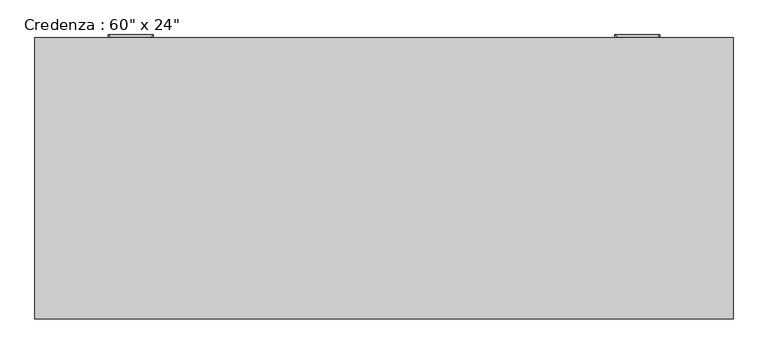
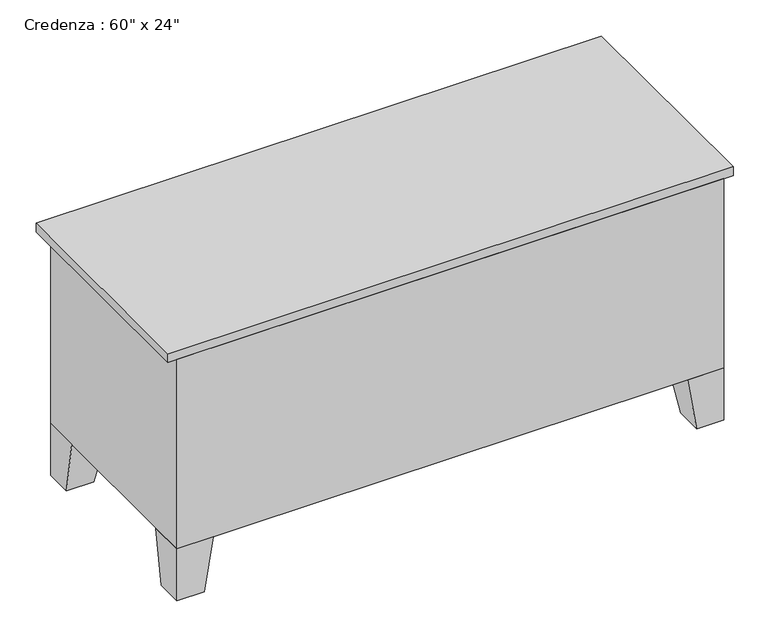
"""IFC4 building model written with IfcOpenShell, lengths in millimetres: furniture geometry."""

from ifc_helpers import new_model, si_unit, frame, origin, place, context, project, spatial, polyline, outline, extrude, faceted_brep, source, transform, mapped, element, save


def furniture_2f1724fb(model_context):
    return source(origin(), model_context, "Body", "SolidModel", [
        extrude(outline(polyline([(455.5023176, 267.2714583), (455.5023176, 254.5714583), (46.8442623, 254.5714583), (46.8442623, 267.2714583), (455.5023176, 267.2714583)])), frame((0.0, 0.0, 171.45), z_axis=(0.0, 0.0, 1.0), x_axis=(1.0, 0.0, 0.0)), (0.0, 0.0, 1.0), 520.7),
        extrude(outline(polyline([(73.6254475, 279.9714583), (73.6254475, 267.2714583), (-302.4057377, 267.2714583), (-302.4057377, 279.9714583), (73.6254475, 279.9714583)])), frame((0.0, 0.0, 171.45), z_axis=(0.0, 0.0, 1.0), x_axis=(1.0, 0.0, 0.0)), (0.0, 0.0, 1.0), 520.7),
        faceted_brep([(719.9442623, -309.3803279, 152.4), (821.5442623, -309.3803279, 152.4), (821.5442623, -207.7803279, 152.4), (719.9442623, -207.7803279, 152.4), (745.3442623, -309.3803279, 0.0), (745.3442623, -233.1803279, 0.0), (821.5442623, -233.1803279, 0.0), (821.5442623, -309.3803279, 0.0)], [[[0, 1, 2, 3]], [[4, 5, 6, 7]], [[4, 0, 3, 5]], [[5, 3, 2, 6]], [[6, 2, 1, 7]], [[7, 1, 0, 4]]]),
        extrude(outline(polyline([(802.4942623, 306.5696721), (802.4942623, 300.2196721), (440.5442623, 300.2196721), (440.5442623, 306.5696721), (802.4942623, 306.5696721)])), frame((0.0, 0.0, 584.2), z_axis=(0.0, 0.0, 1.0), x_axis=(1.0, 0.0, 0.0)), (0.0, 0.0, 1.0), 107.95),
        extrude(outline(polyline([(802.4942623, 306.5696721), (802.4942623, 300.2196721), (440.5442623, 300.2196721), (440.5442623, 306.5696721), (802.4942623, 306.5696721)])), frame((0.0, 0.0, 171.45), z_axis=(0.0, 0.0, 1.0), x_axis=(1.0, 0.0, 0.0)), (0.0, 0.0, 1.0), 393.7),
        extrude(outline(polyline([(-321.4557377, 306.5696721), (-321.4557377, 300.2196721), (-683.4057377, 300.2196721), (-683.4057377, 306.5696721), (-321.4557377, 306.5696721)])), frame((0.0, 0.0, 584.2), z_axis=(0.0, 0.0, 1.0), x_axis=(1.0, 0.0, 0.0)), (0.0, 0.0, 1.0), 107.95),
        extrude(outline(polyline([(-321.4557377, 306.5696721), (-321.4557377, 300.2196721), (-683.4057377, 300.2196721), (-683.4057377, 306.5696721), (-321.4557377, 306.5696721)])), frame((0.0, 0.0, 171.45), z_axis=(0.0, 0.0, 1.0), x_axis=(1.0, 0.0, 0.0)), (0.0, 0.0, 1.0), 393.7),
        faceted_brep([(-600.8557377, 300.2196721, 152.4), (-702.4557377, 300.2196721, 152.4), (-702.4557377, 198.6196721, 152.4), (-600.8557377, 198.6196721, 152.4), (-626.2557377, 300.2196721, 0.0), (-626.2557377, 224.0196721, 0.0), (-702.4557377, 224.0196721, 0.0), (-702.4557377, 300.2196721, 0.0)], [[[0, 1, 2, 3]], [[4, 5, 6, 7]], [[4, 0, 3, 5]], [[5, 3, 2, 6]], [[6, 2, 1, 7]], [[7, 1, 0, 4]]]),
        faceted_brep([(-600.8557377, -309.3803279, 152.4), (-600.8557377, -207.7803279, 152.4), (-702.4557377, -207.7803279, 152.4), (-702.4557377, -309.3803279, 152.4), (-626.2557377, -309.3803279, 0.0), (-702.4557377, -309.3803279, 0.0), (-702.4557377, -233.1803279, 0.0), (-626.2557377, -233.1803279, 0.0)], [[[0, 1, 2, 3]], [[4, 5, 6, 7]], [[4, 0, 3, 5]], [[5, 3, 2, 6]], [[6, 2, 1, 7]], [[7, 1, 0, 4]]]),
        faceted_brep([(719.9442623, 300.2196721, 152.4), (719.9442623, 198.6196721, 152.4), (821.5442623, 198.6196721, 152.4), (821.5442623, 300.2196721, 152.4), (745.3442623, 300.2196721, 0.0), (821.5442623, 300.2196721, 0.0), (821.5442623, 224.0196721, 0.0), (745.3442623, 224.0196721, 0.0)], [[[0, 1, 2, 3]], [[4, 5, 6, 7]], [[4, 0, 3, 5]], [[5, 3, 2, 6]], [[6, 2, 1, 7]], [[7, 1, 0, 4]]]),
        faceted_brep([(821.5442623, -309.3803279, 711.2), (821.5442623, 300.2196721, 711.2), (-702.4557377, 300.2196721, 711.2), (-702.4557377, -309.3803279, 711.2), (821.5442623, -309.3803279, 152.4), (-702.4557377, -309.3803279, 152.4), (-702.4557377, 300.2196721, 152.4), (821.5442623, 300.2196721, 152.4), (-302.4057377, 300.2196721, 692.15), (-302.4057377, 300.2196721, 171.45), (421.4942623, 300.2196721, 171.45), (421.4942623, 300.2196721, 692.15), (421.4942623, -290.3303279, 692.15), (421.4942623, -290.3303279, 171.45), (-302.4057377, -290.3303279, 171.45), (-302.4057377, -290.3303279, 692.15)], [[[0, 1, 2, 3]], [[4, 5, 6, 7]], [[3, 5, 4, 0]], [[2, 6, 5, 3]], [[1, 7, 6, 2], [8, 9, 10, 11]], [[0, 4, 7, 1]], [[12, 13, 14, 15]], [[15, 8, 11, 12]], [[14, 9, 8, 15]], [[13, 10, 9, 14]], [[12, 11, 10, 13]]]),
        extrude(outline(polyline([(846.9442623, -309.3803279), (-727.8557377, -309.3803279), (-727.8557377, 325.6196721), (846.9442623, 325.6196721), (846.9442623, -309.3803279)])), frame((0.0, 0.0, 711.2), z_axis=(0.0, 0.0, 1.0), x_axis=(1.0, 0.0, 0.0)), (0.0, 0.0, 1.0), 25.4),
        faceted_brep([(-556.4057377, 306.5696721, 527.05), (-562.7557377, 306.5696721, 527.05), (-562.7557377, 306.5696721, 514.35), (-556.4057377, 306.5696721, 514.35), (-556.4057377, 325.6196721, 514.35), (-556.4057377, 325.6196721, 527.05), (-562.7557377, 331.9696721, 514.35), (-562.7557377, 331.9696721, 527.05), (-467.5057377, 325.6196721, 514.35), (-467.5057377, 325.6196721, 527.05), (-461.1557377, 331.9696721, 514.35), (-461.1557377, 331.9696721, 527.05), (-467.5057377, 306.5696721, 527.05), (-467.5057377, 306.5696721, 514.35), (-461.1557377, 306.5696721, 514.35), (-461.1557377, 306.5696721, 527.05)], [[[0, 1, 2, 3]], [[3, 4, 5, 0]], [[2, 6, 4, 3]], [[1, 7, 6, 2]], [[0, 5, 7, 1]], [[4, 8, 9, 5]], [[6, 10, 8, 4]], [[7, 11, 10, 6]], [[5, 9, 11, 7]], [[12, 13, 14, 15]], [[8, 13, 12, 9]], [[10, 14, 13, 8]], [[11, 15, 14, 10]], [[9, 12, 15, 11]]]),
        faceted_brep([(-556.4057377, 306.5696721, 654.05), (-562.7557377, 306.5696721, 654.05), (-562.7557377, 306.5696721, 641.35), (-556.4057377, 306.5696721, 641.35), (-556.4057377, 325.6196721, 641.35), (-556.4057377, 325.6196721, 654.05), (-562.7557377, 331.9696721, 641.35), (-562.7557377, 331.9696721, 654.05), (-467.5057377, 325.6196721, 641.35), (-467.5057377, 325.6196721, 654.05), (-461.1557377, 331.9696721, 641.35), (-461.1557377, 331.9696721, 654.05), (-467.5057377, 306.5696721, 654.05), (-467.5057377, 306.5696721, 641.35), (-461.1557377, 306.5696721, 641.35), (-461.1557377, 306.5696721, 654.05)], [[[0, 1, 2, 3]], [[3, 4, 5, 0]], [[2, 6, 4, 3]], [[1, 7, 6, 2]], [[0, 5, 7, 1]], [[4, 8, 9, 5]], [[6, 10, 8, 4]], [[7, 11, 10, 6]], [[5, 9, 11, 7]], [[12, 13, 14, 15]], [[8, 13, 12, 9]], [[10, 14, 13, 8]], [[11, 15, 14, 10]], [[9, 12, 15, 11]]]),
        faceted_brep([(586.5942623, 306.5696721, 654.1373112), (580.2442623, 306.5696721, 654.1373112), (580.2442623, 306.5696721, 641.4373112), (586.5942623, 306.5696721, 641.4373112), (586.5942623, 325.6196721, 641.4373112), (586.5942623, 325.6196721, 654.1373112), (580.2442623, 331.9696721, 641.4373112), (580.2442623, 331.9696721, 654.1373112), (675.4942623, 325.6196721, 641.4373112), (675.4942623, 325.6196721, 654.1373112), (681.8442623, 331.9696721, 641.4373112), (681.8442623, 331.9696721, 654.1373112), (675.4942623, 306.5696721, 654.1373112), (675.4942623, 306.5696721, 641.4373112), (681.8442623, 306.5696721, 641.4373112), (681.8442623, 306.5696721, 654.1373112)], [[[0, 1, 2, 3]], [[3, 4, 5, 0]], [[2, 6, 4, 3]], [[1, 7, 6, 2]], [[0, 5, 7, 1]], [[4, 8, 9, 5]], [[6, 10, 8, 4]], [[7, 11, 10, 6]], [[5, 9, 11, 7]], [[12, 13, 14, 15]], [[8, 13, 12, 9]], [[10, 14, 13, 8]], [[11, 15, 14, 10]], [[9, 12, 15, 11]]]),
        faceted_brep([(586.5942623, 306.5696721, 527.05), (580.2442623, 306.5696721, 527.05), (580.2442623, 306.5696721, 514.35), (586.5942623, 306.5696721, 514.35), (586.5942623, 325.6196721, 514.35), (586.5942623, 325.6196721, 527.05), (580.2442623, 331.9696721, 514.35), (580.2442623, 331.9696721, 527.05), (675.4942623, 325.6196721, 514.35), (675.4942623, 325.6196721, 527.05), (681.8442623, 331.9696721, 514.35), (681.8442623, 331.9696721, 527.05), (675.4942623, 306.5696721, 527.05), (675.4942623, 306.5696721, 514.35), (681.8442623, 306.5696721, 514.35), (681.8442623, 306.5696721, 527.05)], [[[0, 1, 2, 3]], [[3, 4, 5, 0]], [[2, 6, 4, 3]], [[1, 7, 6, 2]], [[0, 5, 7, 1]], [[4, 8, 9, 5]], [[6, 10, 8, 4]], [[7, 11, 10, 6]], [[5, 9, 11, 7]], [[12, 13, 14, 15]], [[8, 13, 12, 9]], [[10, 14, 13, 8]], [[11, 15, 14, 10]], [[9, 12, 15, 11]]]),
    ])


if __name__ == "__main__":
    model = new_model("IFC4")
    model_context = context("Model", 3, world=origin())
    ifc_project = project(units=[si_unit("LENGTHUNIT", "METRE", prefix="MILLI")], contexts=[model_context])
    site = spatial("IfcSite", under=ifc_project)
    building = spatial("IfcBuilding", under=site)
    placement = place(None, origin())
    furniture_shape = furniture_2f1724fb(model_context)
    element("IfcFurniture", 1, ObjectType="Credenza : 60\" x 24\"", at=placement, inside=building, context=model_context, shape_type="MappedRepresentation", body=[
        mapped(furniture_shape, transform((0.0, 0.0, 0.0), x_axis=(1.0, 0.0, 0.0), y_axis=(0.0, 1.0, 0.0), z_axis=(0.0, 0.0, 1.0))),
    ])
    save(model, "model.ifc")

# Revit data of these elements
# Type "Credenza : 60\" x 24\""
#   Assembly Code = "E2020200"
#   Depth = 2' - 0"
#   Height = 2' - 5"
#   Width = 5' - 0"
#   Body Material = Laminate, Ivory, Matte
#   Handles/Legs Material = Steel, Chrome Plated
#   Top Material = Cherry
#   Default Elevation = 0
# Element 1 (IfcFurniture, "Credenza : 60\" x 24\"")
#   Materials on its faces: "Steel, Chrome Plated", "Laminate, Ivory, Matte", "Cherry"
# Materials
#   "Laminate, Ivory, Matte": class "Plastic", colour RGB 247 247 239, transparency 0, Description = "Plastic Laminate - Ivory, Matte", Cost = 0
#   "Steel, Chrome Plated": class "Metal", colour RGB 17 17 17, transparency 0, Description = "Chromiuim plated steel", Cost = 0
#   "Cherry": class "Wood", colour RGB 226 177 128, transparency 0, Description = "Prunus Serotina", Cost = 0
